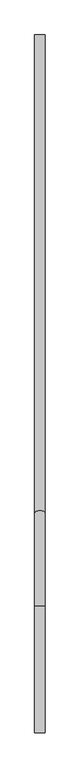
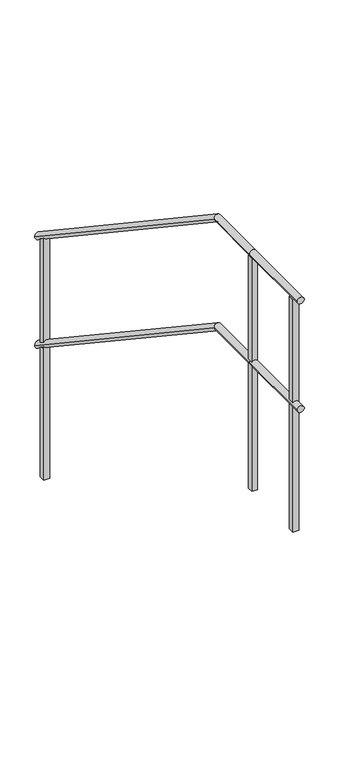
"""IFC4 building model written with IfcOpenShell, lengths in millimetres: railing geometry."""

from ifc_helpers import new_model, si_unit, frame, origin, place, context, project, spatial, polyline, circle_curve, ellipse_curve, outline, extrude, source, transform, mapped, element, save
from ifc_brep_helpers import plane_surface, cylinder_surface, advanced_brep


def railing_e8cc59b0(model_context):
    return source(origin(), model_context, "Body", "SolidModel", [
        advanced_brep(
        [(12192.5845799, 439.5208589, 9484.9618634), (12162.5845799, 439.5208589, 9484.9618634), (12192.5845799, 799.5208589, 9484.9618634), (12162.5845799, 799.5208589, 9484.9618634)],
        [
            (0, 1, circle_curve(frame((12177.5845799, 439.5208589, 9484.9618634), z_axis=(0.0, -1.0, 0.0), x_axis=(-1.0, 0.0, 0.0)), 15.0)),
            (1, 0, circle_curve(frame((12177.5845799, 439.5208589, 9484.9618634), z_axis=(0.0, -1.0, 0.0), x_axis=(-1.0, 0.0, 0.0)), 15.0)),
            (2, 3, circle_curve(frame((12177.5845799, 799.5208589, 9484.9618634), z_axis=(0.0, 1.0, 0.0), x_axis=(-1.0, 0.0, 0.0)), 15.0)),
            (3, 2, circle_curve(frame((12177.5845799, 799.5208589, 9484.9618634), z_axis=(0.0, 1.0, 0.0), x_axis=(-1.0, 0.0, 0.0)), 15.0)),
            (1, 3),
            (2, 0),
        ],
        [
            plane_surface(frame((12177.5845799, 439.5208589, 9499.9618634), z_axis=(0.0, -1.0, 0.0), x_axis=(0.0, 0.0, 1.0))),
            plane_surface(frame((12177.5845799, 799.5208589, 9499.9618634), z_axis=(0.0, 1.0, 0.0), x_axis=(0.0, 0.0, 1.0))),
            cylinder_surface(frame((12177.5845799, 439.5208589, 9484.9618634), z_axis=(0.0, -1.0, 0.0), x_axis=(-1.0, 0.0, 0.0)), 15.0),
        ],
        [
            (0, [[1, 2]]),
            (1, [[3, 4]]),
            (2, [[-2, 5, -3, 6]]),
            (2, [[-1, -6, -4, -5]]),
        ],
    ),
        advanced_brep(
        [(12192.5845799, 799.5208589, 9484.9618634), (12162.5845799, 799.5208589, 9484.9618634), (12162.5845799, 1064.9792243, 9484.9618634), (12192.5845799, 1064.9792243, 9484.9618634), (12192.5845799, 2419.5208589, 8581.934107), (12162.5845799, 2419.5208589, 8581.934107)],
        [
            (0, 1, circle_curve(frame((12177.5845799, 799.5208589, 9484.9618634), z_axis=(0.0, -1.0, 0.0), x_axis=(-1.0, 0.0, 0.0)), 15.0)),
            (1, 0, circle_curve(frame((12177.5845799, 799.5208589, 9484.9618634), z_axis=(0.0, -1.0, 0.0), x_axis=(-1.0, 0.0, 0.0)), 15.0)),
            (1, 2),
            (2, 3, ellipse_curve(frame((12177.5845799, 1064.9792243, 9484.9618634), z_axis=(0.0, -0.9570920264890528, 0.28978414868843017), x_axis=(0.0, -0.2897841486884305, -0.9570920264890528)), 15.6724741, 15.0)),
            (3, 0),
            (3, 2, ellipse_curve(frame((12177.5845799, 1064.9792243, 9484.9618634), z_axis=(0.0, -0.9570920264890528, 0.28978414868843017), x_axis=(0.0, -0.2897841486884305, -0.9570920264890528)), 15.6724741, 15.0)),
            (4, 5, ellipse_curve(frame((12177.5845799, 2419.5208589, 8581.934107), z_axis=(0.0, 1.0, 0.0), x_axis=(0.0, 0.0, 1.0)), 18.0277564, 15.0)),
            (5, 4, ellipse_curve(frame((12177.5845799, 2419.5208589, 8581.934107), z_axis=(0.0, 1.0, 0.0), x_axis=(0.0, 0.0, 1.0)), 18.0277564, 15.0)),
            (2, 5),
            (4, 3),
        ],
        [
            plane_surface(frame((12177.5845799, 799.5208589, 9499.9618634), z_axis=(0.0, -1.0, 0.0), x_axis=(0.0, 0.0, 1.0))),
            cylinder_surface(frame((12177.5845799, 799.5208589, 9484.9618634), z_axis=(0.0, -1.0, 0.0), x_axis=(-1.0, 0.0, 0.0)), 15.0),
            plane_surface(frame((12177.5845799, 2419.5208589, 8599.9618634), z_axis=(0.0, 1.0, 0.0), x_axis=(0.0, 0.0, 1.0))),
            cylinder_surface(frame((12177.5845799, 1061.2003559, 9487.481109), z_axis=(0.0, -0.8320502943378436, 0.5547001962252293), x_axis=(-1.0, 0.0, 0.0)), 15.0),
        ],
        [
            (0, [[1, 2]]),
            (1, [[-2, 3, 4, 5]]),
            (1, [[-1, -5, 6, -3]]),
            (2, [[7, 8]]),
            (3, [[-4, 9, -7, 10]]),
            (3, [[-6, -10, -8, -9]]),
        ],
    ),
        advanced_brep(
        [(12192.5845799, 439.5208589, 9984.9618634), (12162.5845799, 439.5208589, 9984.9618634), (12192.5845799, 799.5208589, 9984.9618634), (12162.5845799, 799.5208589, 9984.9618634)],
        [
            (0, 1, circle_curve(frame((12177.5845799, 439.5208589, 9984.9618634), z_axis=(0.0, -1.0, 0.0), x_axis=(-1.0, 0.0, 0.0)), 15.0)),
            (1, 0, circle_curve(frame((12177.5845799, 439.5208589, 9984.9618634), z_axis=(0.0, -1.0, 0.0), x_axis=(-1.0, 0.0, 0.0)), 15.0)),
            (2, 3, circle_curve(frame((12177.5845799, 799.5208589, 9984.9618634), z_axis=(0.0, 1.0, 0.0), x_axis=(-1.0, 0.0, 0.0)), 15.0)),
            (3, 2, circle_curve(frame((12177.5845799, 799.5208589, 9984.9618634), z_axis=(0.0, 1.0, 0.0), x_axis=(-1.0, 0.0, 0.0)), 15.0)),
            (1, 3),
            (2, 0),
        ],
        [
            plane_surface(frame((12177.5845799, 439.5208589, 9999.9618634), z_axis=(0.0, -1.0, 0.0), x_axis=(0.0, 0.0, 1.0))),
            plane_surface(frame((12177.5845799, 799.5208589, 9999.9618634), z_axis=(0.0, 1.0, 0.0), x_axis=(0.0, 0.0, 1.0))),
            cylinder_surface(frame((12177.5845799, 439.5208589, 9984.9618634), z_axis=(0.0, -1.0, 0.0), x_axis=(-1.0, 0.0, 0.0)), 15.0),
        ],
        [
            (0, [[1, 2]]),
            (1, [[3, 4]]),
            (2, [[-2, 5, -3, 6]]),
            (2, [[-1, -6, -4, -5]]),
        ],
    ),
        advanced_brep(
        [(12192.5845799, 799.5208589, 9984.9618634), (12162.5845799, 799.5208589, 9984.9618634), (12162.5845799, 1064.9792243, 9984.9618634), (12192.5845799, 1064.9792243, 9984.9618634), (12192.5845799, 2419.5208589, 9081.934107), (12162.5845799, 2419.5208589, 9081.934107)],
        [
            (0, 1, circle_curve(frame((12177.5845799, 799.5208589, 9984.9618634), z_axis=(0.0, -1.0, 0.0), x_axis=(-1.0, 0.0, 0.0)), 15.0)),
            (1, 0, circle_curve(frame((12177.5845799, 799.5208589, 9984.9618634), z_axis=(0.0, -1.0, 0.0), x_axis=(-1.0, 0.0, 0.0)), 15.0)),
            (1, 2),
            (2, 3, ellipse_curve(frame((12177.5845799, 1064.9792243, 9984.9618634), z_axis=(0.0, -0.9570920264890528, 0.28978414868843017), x_axis=(0.0, -0.2897841486884305, -0.9570920264890528)), 15.6724741, 15.0)),
            (3, 0),
            (3, 2, ellipse_curve(frame((12177.5845799, 1064.9792243, 9984.9618634), z_axis=(0.0, -0.9570920264890528, 0.28978414868843017), x_axis=(0.0, -0.2897841486884305, -0.9570920264890528)), 15.6724741, 15.0)),
            (4, 5, ellipse_curve(frame((12177.5845799, 2419.5208589, 9081.934107), z_axis=(0.0, 1.0, 0.0), x_axis=(0.0, 0.0, 1.0)), 18.0277564, 15.0)),
            (5, 4, ellipse_curve(frame((12177.5845799, 2419.5208589, 9081.934107), z_axis=(0.0, 1.0, 0.0), x_axis=(0.0, 0.0, 1.0)), 18.0277564, 15.0)),
            (2, 5),
            (4, 3),
        ],
        [
            plane_surface(frame((12177.5845799, 799.5208589, 9999.9618634), z_axis=(0.0, -1.0, 0.0), x_axis=(0.0, 0.0, 1.0))),
            cylinder_surface(frame((12177.5845799, 799.5208589, 9984.9618634), z_axis=(0.0, -1.0, 0.0), x_axis=(-1.0, 0.0, 0.0)), 15.0),
            plane_surface(frame((12177.5845799, 2419.5208589, 9099.9618634), z_axis=(0.0, 1.0, 0.0), x_axis=(0.0, 0.0, 1.0))),
            cylinder_surface(frame((12177.5845799, 1061.2003559, 9987.481109), z_axis=(0.0, -0.8320502943378436, 0.5547001962252293), x_axis=(-1.0, 0.0, 0.0)), 15.0),
        ],
        [
            (0, [[1, 2]]),
            (1, [[-2, 3, 4, 5]]),
            (1, [[-1, -5, 6, -3]]),
            (2, [[7, 8]]),
            (3, [[-4, 9, -7, 10]]),
            (3, [[-6, -10, -8, -9]]),
        ],
    ),
        extrude(outline(polyline([(12165.0845799, 787.0208589), (12165.0845799, 812.0208589), (12190.0845799, 812.0208589), (12190.0845799, 787.0208589), (12165.0845799, 787.0208589)])), frame((0.0, 0.0, 8899.9618634), z_axis=(0.0, 0.0, 1.0), x_axis=(1.0, 0.0, 0.0)), (0.0, 0.0, 1.0), 1070.0),
        extrude(outline(polyline([(2357.0208589, 9111.62853), (2382.0208589, 9094.9618634), (2382.0208589, 7999.9618634), (2357.0208589, 7999.9618634), (2357.0208589, 9111.62853)])), frame((12165.0845799, 0.0, 0.0), z_axis=(1.0, 0.0, 0.0), x_axis=(0.0, 1.0, 0.0)), (0.0, 0.0, 1.0), 25.0),
        extrude(outline(polyline([(12165.0845799, 477.0208589), (12165.0845799, 502.0208589), (12190.0845799, 502.0208589), (12190.0845799, 477.0208589), (12165.0845799, 477.0208589)])), frame((0.0, 0.0, 8899.9618634), z_axis=(0.0, 0.0, 1.0), x_axis=(1.0, 0.0, 0.0)), (0.0, 0.0, 1.0), 1070.0),
    ])


if __name__ == "__main__":
    model = new_model("IFC4")
    model_context = context("Model", 3, world=origin())
    ifc_project = project(units=[si_unit("LENGTHUNIT", "METRE", prefix="MILLI")], contexts=[model_context])
    site = spatial("IfcSite", under=ifc_project)
    building = spatial("IfcBuilding", under=site)
    placement = place(None, origin())
    railing_shape = railing_e8cc59b0(model_context)
    element("IfcRailing", 1, at=placement, inside=building, context=model_context, shape_type="MappedRepresentation", body=[
        mapped(railing_shape, transform((0.0, 0.0, 0.0), x_axis=(1.0, 0.0, 0.0), y_axis=(0.0, 1.0, 0.0), z_axis=(0.0, 0.0, 1.0))),
    ])
    save(model, "model.ifc")
